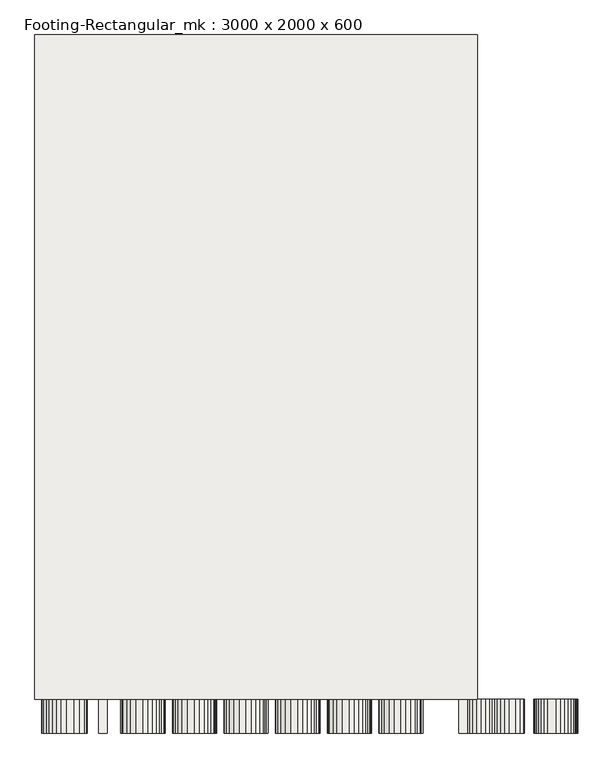
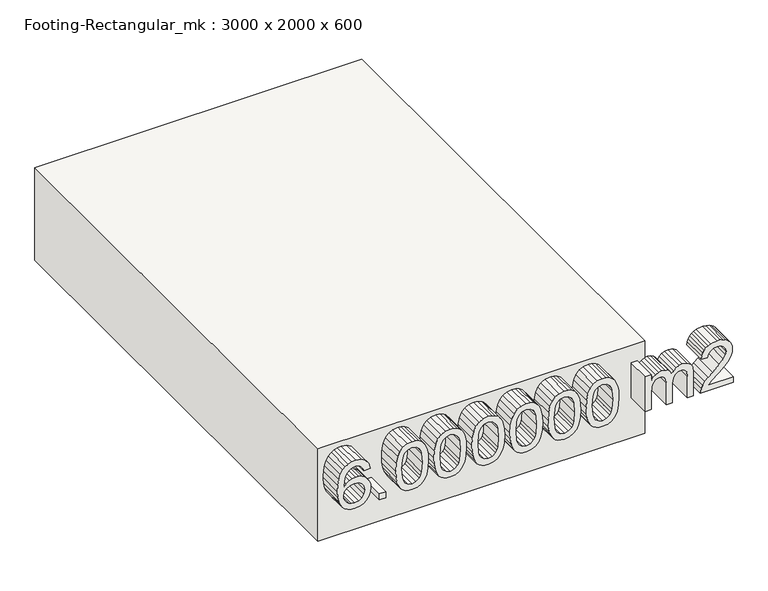
"""IFC4 building model written with IfcOpenShell, lengths in millimetres: slab geometry, Footing-Rectangular_mk : 3000 x 2000 x 600."""

from ifc_helpers import new_model, si_unit, frame, origin, place, context, project, spatial, polyline, outline, extrude, source, transform, mapped, element, save


def footing_rectangular_mk_3000_x_2000_x_600_52bbaf05(model_context):
    return source(origin(), model_context, "Body", "SweptSolid", [
        extrude(outline(polyline([(1000.0, 2085.6), (1000.0, -914.4), (-1000.0, -914.4), (-1000.0, 2085.6), (1000.0, 2085.6)])), frame((0.0, 0.0, -600.0), z_axis=(0.0, 0.0, 1.0), x_axis=(1.0, 0.0, 0.0)), (0.0, 0.0, 1.0), 600.0),
        extrude(outline(polyline([(-113.8433338, -768.5560264), (-80.0293968, -777.9250337), (-54.4319304, -796.6630483), (-38.3150072, -823.4130513), (-32.9426994, -856.8180237), (-35.1130002, -880.170832), (-41.6239026, -901.0047902), (-52.4754066, -919.3198982), (-67.6675122, -935.116156), (-90.5927666, -949.6901673), (-119.5130704, -960.1001754), (-154.4284234, -966.3461803), (-195.3388258, -968.4281819), (-231.829622, -966.5529863), (-262.7808068, -960.9273993), (-288.1923801, -951.551421), (-308.064342, -938.4250514), (-323.0287287, -922.3243938), (-333.7175763, -904.0255515), (-340.1308848, -883.5285244), (-342.2686543, -860.8333125), (-339.0434108, -834.417917), (-329.36768, -810.9396308), (-313.6225428, -791.2907406), (-292.1890797, -776.3635325), (-266.9169261, -766.9387573), (-239.6557174, -763.7971656), (-219.1563666, -765.4655553), (-200.6367763, -770.4707244), (-184.0969465, -778.8126728), (-169.5368771, -790.4914006), (-157.6629616, -804.5449116), (-149.1815934, -820.0112093), (-144.0927725, -836.8902939), (-142.3964989, -855.1821653), (-144.8781704, -876.4762086), (-152.3231852, -896.785019), (-164.8802574, -915.0861851), (-182.6981016, -930.3572952), (-143.2051334, -927.4294804), (-114.847156, -919.5383225), (-94.7985958, -907.8549473), (-80.2338791, -893.5504808), (-73.3186594, -876.8944679), (-71.0135862, -859.1974541), (-74.9731071, -838.32167), (-86.8516699, -821.0522101), (-99.734055, -812.7613823), (-118.6021946, -806.6269132), (-113.8433338, -768.5560264)]), holes=[polyline([(-239.0608598, -930.3572952), (-215.3316181, -925.6263183), (-196.6400768, -911.4333876), (-184.5105584, -890.4553623), (-180.4673856, -865.3691017), (-184.5105584, -838.7956971), (-196.6400768, -818.7099583), (-215.7963506, -806.0785288), (-240.9197898, -801.8680524), (-267.0935244, -806.1342967), (-287.1699686, -818.9330299), (-299.9408179, -838.6841613), (-304.1977676, -863.8076005), (-302.1436499, -882.2388917), (-295.9812969, -898.1234487), (-285.8873069, -911.2846732), (-272.0382783, -921.5459669), (-255.9306497, -928.1544631), (-239.0608598, -930.3572952)])]), frame((0.0, -1066.8, 0.0), z_axis=(0.0, 1.0, 0.0), x_axis=(0.0, 0.0, 1.0)), (0.0, 0.0, 1.0), 152.4),
        extrude(outline(polyline([(-673.3788095, -1066.8), (-711.4496963, -1066.8), (-711.4496963, -914.4), (-673.3788095, -914.4), (-673.3788095, -1066.8)])), frame((0.0, 0.0, -337.5097935), z_axis=(0.0, 0.0, 1.0), x_axis=(1.0, 0.0, 0.0)), (0.0, 0.0, 1.0), 38.0708868),
        extrude(outline(polyline([(-187.6800341, -611.5136186), (-227.540141, -609.6175099), (-261.7583953, -603.9291841), (-290.334797, -594.448641), (-313.2693461, -581.1758807), (-325.9565434, -567.3454413), (-335.0188273, -551.1355716), (-340.4561976, -532.5462714), (-342.2686543, -511.5775408), (-338.0953565, -480.8029544), (-325.5754628, -455.8468189), (-304.5695536, -436.5418307), (-274.9382091, -422.720686), (-236.1516343, -414.4112688), (-187.6800341, -411.6414631), (-147.2947795, -413.370268), (-116.1112284, -418.5566827), (-91.5547629, -426.4757246), (-71.0507648, -436.4024109), (-54.7386539, -449.5450461), (-42.7578499, -467.1119348), (-35.3964871, -488.117844), (-32.9426994, -511.5775408), (-37.0881134, -542.1848236), (-49.5243552, -567.0851911), (-70.4466125, -586.4180633), (-100.0500731, -600.3228599), (-138.9295944, -608.7159289), (-187.6800341, -611.5136186)]), holes=[polyline([(-187.6056769, -573.4427318), (-128.4917023, -568.8325854), (-107.1883643, -563.0699023), (-91.3874592, -555.002146), (-76.1070544, -535.8551668), (-71.0135862, -512.023684), (-76.7948585, -486.8537716), (-94.1386756, -466.9632204), (-108.6522717, -459.4159645), (-129.0679706, -454.0250675), (-187.6056769, -449.7123498), (-247.3981609, -454.1737819), (-267.8765987, -459.7505719), (-282.0765004, -467.558078), (-298.6674508, -487.4858078), (-304.1977676, -511.5775408), (-298.6860401, -535.6692738), (-282.1508576, -555.5970036), (-267.9741925, -563.4045097), (-247.4911074, -568.9812998), (-187.6056769, -573.4427318)])]), frame((0.0, -1066.8, 0.0), z_axis=(0.0, 1.0, 0.0), x_axis=(0.0, 0.0, 1.0)), (0.0, 0.0, 1.0), 152.4),
        extrude(outline(polyline([(-187.6800341, -378.3294372), (-227.540141, -376.4333285), (-261.7583953, -370.7450027), (-290.334797, -361.2644596), (-313.2693461, -347.9916993), (-325.9565434, -334.1612599), (-335.0188273, -317.9513902), (-340.4561976, -299.36209), (-342.2686543, -278.3933594), (-338.0953565, -247.618773), (-325.5754628, -222.6626375), (-304.5695536, -203.3576493), (-274.9382091, -189.5365046), (-236.1516343, -181.2270874), (-187.6800341, -178.4572817), (-147.2947795, -180.1860866), (-116.1112284, -185.3725013), (-91.5547629, -193.2915432), (-71.0507648, -203.2182295), (-54.7386539, -216.3608647), (-42.7578499, -233.9277534), (-35.3964871, -254.9336626), (-32.9426994, -278.3933594), (-37.0881134, -309.0006422), (-49.5243552, -333.9010097), (-70.4466125, -353.2338819), (-100.0500731, -367.1386785), (-138.9295944, -375.5317475), (-187.6800341, -378.3294372)]), holes=[polyline([(-187.6056769, -340.2585504), (-128.4917023, -335.648404), (-107.1883643, -329.8857209), (-91.3874592, -321.8179646), (-76.1070544, -302.6709855), (-71.0135862, -278.8395026), (-76.7948585, -253.6695902), (-94.1386756, -233.779039), (-108.6522717, -226.2317831), (-129.0679706, -220.8408861), (-187.6056769, -216.5281684), (-247.3981609, -220.9896005), (-267.8765987, -226.5663905), (-282.0765004, -234.3738966), (-298.6674508, -254.3016264), (-304.1977676, -278.3933594), (-298.6860401, -302.4850924), (-282.1508576, -322.4128222), (-267.9741925, -330.2203283), (-247.4911074, -335.7971184), (-187.6056769, -340.2585504)])]), frame((0.0, -1066.8, 0.0), z_axis=(0.0, 1.0, 0.0), x_axis=(0.0, 0.0, 1.0)), (0.0, 0.0, 1.0), 152.4),
        extrude(outline(polyline([(-187.6800341, -145.1452558), (-227.540141, -143.2491471), (-261.7583953, -137.5608213), (-290.334797, -128.0802782), (-313.2693461, -114.8075179), (-325.9565434, -100.9770786), (-335.0188273, -84.7672088), (-340.4561976, -66.1779086), (-342.2686543, -45.209178), (-338.0953565, -14.4345916), (-325.5754628, 10.5215439), (-304.5695536, 29.8265321), (-274.9382091, 43.6476768), (-236.1516343, 51.957094), (-187.6800341, 54.7268997), (-147.2947795, 52.9980948), (-116.1112284, 47.8116801), (-91.5547629, 39.8926382), (-71.0507648, 29.9659519), (-54.7386539, 16.8233167), (-42.7578499, -0.743572), (-35.3964871, -21.7494812), (-32.9426994, -45.209178), (-37.0881134, -75.8164608), (-49.5243552, -100.7168283), (-70.4466125, -120.0497005), (-100.0500731, -133.9544971), (-138.9295944, -142.3475661), (-187.6800341, -145.1452558)]), holes=[polyline([(-187.6056769, -107.074369), (-128.4917023, -102.4642226), (-107.1883643, -96.7015395), (-91.3874592, -88.6337832), (-76.1070544, -69.4868041), (-71.0135862, -45.6553212), (-76.7948585, -20.4854088), (-94.1386756, -0.5948576), (-108.6522717, 6.9523983), (-129.0679706, 12.3432953), (-187.6056769, 16.656013), (-247.3981609, 12.1945809), (-267.8765987, 6.6177909), (-282.0765004, -1.1897152), (-298.6674508, -21.117445), (-304.1977676, -45.209178), (-298.6860401, -69.3009111), (-282.1508576, -89.2286408), (-267.9741925, -97.0361469), (-247.4911074, -102.612937), (-187.6056769, -107.074369)])]), frame((0.0, -1066.8, 0.0), z_axis=(0.0, 1.0, 0.0), x_axis=(0.0, 0.0, 1.0)), (0.0, 0.0, 1.0), 152.4),
        extrude(outline(polyline([(-187.6800341, 88.0389256), (-227.540141, 89.9350342), (-261.7583953, 95.6233601), (-290.334797, 105.1039032), (-313.2693461, 118.3766635), (-325.9565434, 132.2071028), (-335.0188273, 148.4169726), (-340.4561976, 167.0062728), (-342.2686543, 187.9750034), (-338.0953565, 218.7495898), (-325.5754628, 243.7057253), (-304.5695536, 263.0107135), (-274.9382091, 276.8318582), (-236.1516343, 285.1412754), (-187.6800341, 287.9110811), (-147.2947795, 286.1822762), (-116.1112284, 280.9958614), (-91.5547629, 273.0768196), (-71.0507648, 263.1501333), (-54.7386539, 250.0074981), (-42.7578499, 232.4406094), (-35.3964871, 211.4347002), (-32.9426994, 187.9750034), (-37.0881134, 157.3677206), (-49.5243552, 132.467353), (-70.4466125, 113.1344809), (-100.0500731, 99.2296843), (-138.9295944, 90.8366153), (-187.6800341, 88.0389256)]), holes=[polyline([(-187.6056769, 126.1098124), (-128.4917023, 130.7199588), (-107.1883643, 136.4826419), (-91.3874592, 144.5503982), (-76.1070544, 163.6973773), (-71.0135862, 187.5288602), (-76.7948585, 212.6987726), (-94.1386756, 232.5893238), (-108.6522717, 240.1365797), (-129.0679706, 245.5274767), (-187.6056769, 249.8401944), (-247.3981609, 245.3787623), (-267.8765987, 239.8019723), (-282.0765004, 231.9944662), (-298.6674508, 212.0667364), (-304.1977676, 187.9750034), (-298.6860401, 163.8832703), (-282.1508576, 143.9555406), (-267.9741925, 136.1480345), (-247.4911074, 130.5712444), (-187.6056769, 126.1098124)])]), frame((0.0, -1066.8, 0.0), z_axis=(0.0, 1.0, 0.0), x_axis=(0.0, 0.0, 1.0)), (0.0, 0.0, 1.0), 152.4),
        extrude(outline(polyline([(-187.6800341, 321.223107), (-227.540141, 323.1192156), (-261.7583953, 328.8075415), (-290.334797, 338.2880846), (-313.2693461, 351.5608449), (-325.9565434, 365.3912842), (-335.0188273, 381.601154), (-340.4561976, 400.1904542), (-342.2686543, 421.1591848), (-338.0953565, 451.9337712), (-325.5754628, 476.8899067), (-304.5695536, 496.1948949), (-274.9382091, 510.0160396), (-236.1516343, 518.3254568), (-187.6800341, 521.0952625), (-147.2947795, 519.3664576), (-116.1112284, 514.1800428), (-91.5547629, 506.261001), (-71.0507648, 496.3343147), (-54.7386539, 483.1916795), (-42.7578499, 465.6247908), (-35.3964871, 444.6188816), (-32.9426994, 421.1591848), (-37.0881134, 390.551902), (-49.5243552, 365.6515344), (-70.4466125, 346.3186623), (-100.0500731, 332.4138657), (-138.9295944, 324.0207967), (-187.6800341, 321.223107)]), holes=[polyline([(-187.6056769, 359.2939938), (-128.4917023, 363.9041402), (-107.1883643, 369.6668233), (-91.3874592, 377.7345796), (-76.1070544, 396.8815587), (-71.0135862, 420.7130416), (-76.7948585, 445.882954), (-94.1386756, 465.7735052), (-108.6522717, 473.3207611), (-129.0679706, 478.7116581), (-187.6056769, 483.0243757), (-247.3981609, 478.5629437), (-267.8765987, 472.9861537), (-282.0765004, 465.1786476), (-298.6674508, 445.2509178), (-304.1977676, 421.1591848), (-298.6860401, 397.0674517), (-282.1508576, 377.139722), (-267.9741925, 369.3322159), (-247.4911074, 363.7554258), (-187.6056769, 359.2939938)])]), frame((0.0, -1066.8, 0.0), z_axis=(0.0, 1.0, 0.0), x_axis=(0.0, 0.0, 1.0)), (0.0, 0.0, 1.0), 152.4),
        extrude(outline(polyline([(-187.6800341, 554.4072884), (-227.540141, 556.303397), (-261.7583953, 561.9917229), (-290.334797, 571.472266), (-313.2693461, 584.7450263), (-325.9565434, 598.5754656), (-335.0188273, 614.7853354), (-340.4561976, 633.3746356), (-342.2686543, 654.3433662), (-338.0953565, 685.1179526), (-325.5754628, 710.0740881), (-304.5695536, 729.3790763), (-274.9382091, 743.200221), (-236.1516343, 751.5096382), (-187.6800341, 754.2794439), (-147.2947795, 752.550639), (-116.1112284, 747.3642242), (-91.5547629, 739.4451824), (-71.0507648, 729.5184961), (-54.7386539, 716.3758608), (-42.7578499, 698.8089722), (-35.3964871, 677.803063), (-32.9426994, 654.3433662), (-37.0881134, 623.7360834), (-49.5243552, 598.8357158), (-70.4466125, 579.5028437), (-100.0500731, 565.5980471), (-138.9295944, 557.2049781), (-187.6800341, 554.4072884)]), holes=[polyline([(-187.6056769, 592.4781752), (-128.4917023, 597.0883216), (-107.1883643, 602.8510047), (-91.3874592, 610.918761), (-76.1070544, 630.0657401), (-71.0135862, 653.897223), (-76.7948585, 679.0671354), (-94.1386756, 698.9576866), (-108.6522717, 706.5049425), (-129.0679706, 711.8958395), (-187.6056769, 716.2085571), (-247.3981609, 711.7471251), (-267.8765987, 706.1703351), (-282.0765004, 698.362829), (-298.6674508, 678.4350992), (-304.1977676, 654.3433662), (-298.6860401, 630.2516331), (-282.1508576, 610.3239033), (-267.9741925, 602.5163973), (-247.4911074, 596.9396072), (-187.6056769, 592.4781752)])]), frame((0.0, -1066.8, 0.0), z_axis=(0.0, 1.0, 0.0), x_axis=(0.0, 0.0, 1.0)), (0.0, 0.0, 1.0), 152.4),
        extrude(outline(polyline([(-337.5097935, 916.0807126), (-337.5097935, 954.1515994), (-224.70992, 954.1515994), (-198.5175961, 955.6015648), (-179.2776704, 959.951461), (-165.4100525, 967.5358955), (-155.3346518, 978.6894756), (-149.2001827, 992.2038968), (-147.1553597, 1006.8708547), (-150.2225942, 1024.1310199), (-159.4242978, 1035.7586272), (-174.7790598, 1042.3671234), (-196.3054694, 1044.5699554), (-337.5097935, 1044.5699554), (-337.5097935, 1082.6408422), (-211.2512667, 1082.6408422), (-182.2333691, 1086.3679969), (-162.3985859, 1097.5494609), (-150.9661662, 1114.3634829), (-147.1553597, 1134.9883115), (-148.6425037, 1146.6716866), (-153.1039358, 1156.7377927), (-159.9912715, 1164.5638881), (-168.7561265, 1169.5272312), (-200.5438298, 1173.0591982), (-337.5097935, 1173.0591982), (-337.5097935, 1211.130085), (-184.1852457, 1211.130085), (-150.8639251, 1206.7708941), (-127.4878801, 1193.6933214), (-113.6853247, 1172.5294032), (-109.084473, 1143.9111756), (-111.8496314, 1124.1786334), (-120.1451066, 1106.3979678), (-133.9708986, 1090.5691787), (-153.3270074, 1076.6922661), (-134.6912339, 1068.4014383), (-120.7213749, 1055.7235355), (-111.9936984, 1038.7515045), (-109.084473, 1017.5782916), (-111.9379305, 997.8178655), (-120.4983033, 980.325334), (-133.7431796, 965.6026083), (-150.6501481, 954.1515994), (-113.8433338, 954.1515994), (-113.8433338, 916.0807126), (-337.5097935, 916.0807126)])), frame((0.0, -1066.8, 0.0), z_axis=(0.0, 1.0, 0.0), x_axis=(0.0, 0.0, 1.0)), (0.0, 0.0, 1.0), 152.4),
        extrude(outline(polyline([(-299.4389067, 1453.8319881), (-299.4389067, 1304.2996575), (-280.068856, 1321.4761708), (-243.4479346, 1365.2725621), (-214.1233136, 1398.3150431), (-191.2863583, 1419.8135688), (-172.1579684, 1433.300106), (-153.9590436, 1442.306622), (-136.0668422, 1447.3815009), (-117.8586226, 1449.0731272), (-100.5241002, 1447.504655), (-84.6581325, 1442.7992384), (-70.2607195, 1434.9568774), (-57.3318613, 1423.977572), (-46.661603, 1410.3074654), (-39.0399899, 1394.3927008), (-34.4670221, 1376.2332782), (-32.9426994, 1355.8291976), (-38.426543, 1317.5445339), (-45.2813474, 1301.6437112), (-54.8780736, 1287.9038947), (-67.0865965, 1276.5853346), (-81.776791, 1267.948281), (-98.948657, 1261.9927339), (-118.6021946, 1258.7186935), (-123.3610555, 1296.7895802), (-101.4814492, 1300.9071102), (-84.9183827, 1312.813557), (-74.4897853, 1331.2634374), (-71.0135862, 1355.0112684), (-74.5734372, 1377.625152), (-85.2529901, 1395.4987641), (-101.1003685, 1407.1263714), (-120.1636959, 1411.0022405), (-141.4298553, 1406.8940051), (-163.2908723, 1394.5692991), (-190.2267682, 1369.9198871), (-226.7175645, 1328.8375337), (-250.0192522, 1301.04653), (-270.8485631, 1281.1745681), (-290.7484089, 1267.4370752), (-311.2617017, 1258.0494786), (-337.5097935, 1253.9598326), (-337.5097935, 1453.8319881), (-299.4389067, 1453.8319881)])), frame((0.0, -1066.8, 0.0), z_axis=(0.0, 1.0, 0.0), x_axis=(0.0, 0.0, 1.0)), (0.0, 0.0, 1.0), 152.4),
    ])


if __name__ == "__main__":
    model = new_model("IFC4")
    model_context = context("Model", 3, world=origin())
    ifc_project = project(units=[si_unit("LENGTHUNIT", "METRE", prefix="MILLI")], contexts=[model_context])
    site = spatial("IfcSite", under=ifc_project)
    building = spatial("IfcBuilding", under=site)
    placement = place(None, origin())
    footing_rectangular_mk_3000_x_2000_x_600_shape = footing_rectangular_mk_3000_x_2000_x_600_52bbaf05(model_context)
    element("IfcSlab", 1, ObjectType="Footing-Rectangular_mk : 3000 x 2000 x 600", at=placement, inside=building, context=model_context, shape_type="MappedRepresentation", body=[
        mapped(footing_rectangular_mk_3000_x_2000_x_600_shape, transform((0.0, 0.0, 0.0), x_axis=(1.0, 0.0, 0.0), y_axis=(0.0, 1.0, 0.0), z_axis=(0.0, 0.0, 1.0))),
    ])
    save(model, "model.ifc")

# Revit data of these elements
# Project information
#   Project Issue Date = "Issue Date"
#   Project Status = "Project Status"
#   Client Name = "Owner"
#   Project Address = "Enter address here"
#   Project Name = "Project Name"
#   Project Number = "0001"
# Type "Footing-Rectangular_mk : 3000 x 2000 x 600"
#   ModelText [instance default] = "ModelText"
#   Assembly Code = "A1010100"
#   Width = 2000 mm
#   Length = 3000 mm
#   Foundation Thickness = 600 mm
#   Structural Material [instance default] = Concrete, Cast-in-Place gray
# Element 1 (IfcSlab, "Footing-Rectangular_mk : 3000 x 2000 x 600")
#   ModelText = "6.000000 m2"
#   Materials on its faces: "Concrete, Cast-in-Place gray"
# Materials
#   "Concrete, Cast-in-Place gray": class "Concrete", colour RGB 192 192 192, transparency 0, Description = "Cast-in-place concrete", Cost = 0
